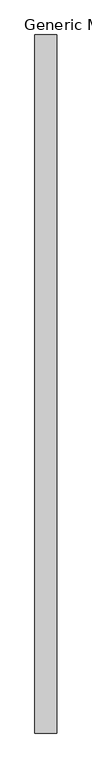
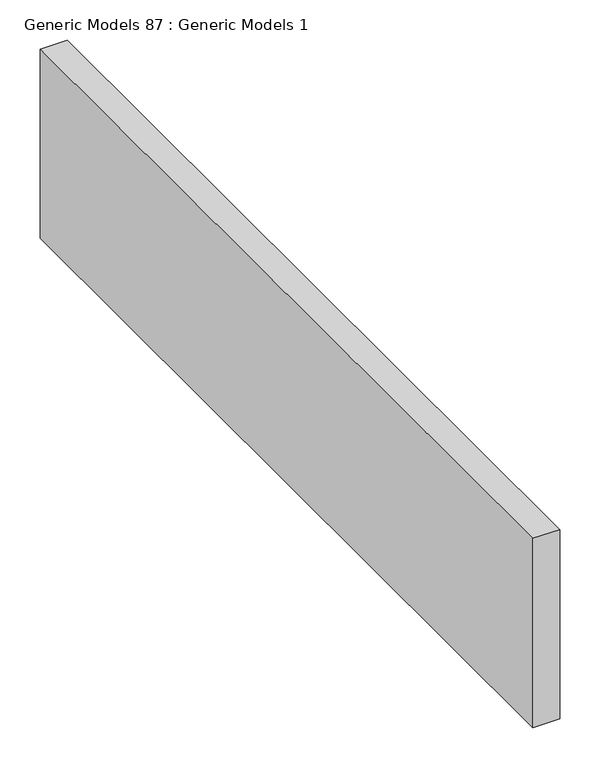
"""IFC4 building model written with IfcOpenShell, lengths in millimetres: proxy geometry, Generic Models 87 : Generic Models 1."""

import ifcopenshell
import ifcopenshell.guid

model = None  # the IFC model being written
_history = None  # IfcOwnerHistory: only IFC2X3 demands one
_inside = {}  # id of a spatial element -> (the spatial element, [elements in it])
_under = {}  # id of a project, library or spatial element -> (it, [spatial elements below it])
_declared = {}  # id of a project -> (the project, [libraries it declares])
_typed = {}  # id of a type object -> (the type object, [elements of that type])
_made_of = {}  # id of a material, layer set ... -> (it, [elements and type objects made of it])


def new_model(schema):
    """Start an empty IFC model of exactly this schema.

    Asked for "IFC4X3", IfcOpenShell would pick the latest addendum, in which some entities
    have other attributes; the version numbers below select the first issue.
    IFC2X3 requires an IfcOwnerHistory on every rooted entity: one is made here for all.
    """
    global model, _history
    if schema == "IFC4X3":
        model = ifcopenshell.file(schema_version=(4, 3, 0, 0))
    else:
        model = ifcopenshell.file(schema=schema)
    _inside.clear()
    _under.clear()
    _declared.clear()
    _typed.clear()
    _made_of.clear()
    _history = None
    if model.schema == "IFC2X3":
        org = make("IfcOrganization", Name="unknown")
        user = make(
            "IfcPersonAndOrganization",
            ThePerson=make("IfcPerson", FamilyName="unknown"),
            TheOrganization=org,
        )
        app = make(
            "IfcApplication",
            ApplicationDeveloper=org,
            Version="unknown",
            ApplicationFullName="unknown",
            ApplicationIdentifier="unknown",
        )
        _history = make(
            "IfcOwnerHistory",
            OwningUser=user,
            OwningApplication=app,
            ChangeAction="ADDED",
            CreationDate=0,
        )
    return model


def make(cls, **values):
    """One entity of the class cls with the attributes given. An attribute that is None is left unset."""
    return model.create_entity(
        cls, **{name: value for name, value in values.items() if value is not None}
    )


def rooted(cls, **values):
    """An entity with a GlobalId (a new one), such as an element, a storey or a relation."""
    return make(cls, GlobalId=ifcopenshell.guid.new(), OwnerHistory=_history, **values)


def si_unit(unit_type, name, prefix=None):
    """IfcSIUnit, for example si_unit("LENGTHUNIT", "METRE", prefix="MILLI")."""
    return make("IfcSIUnit", UnitType=unit_type, Prefix=prefix, Name=name)


def assignment(units):
    """IfcUnitAssignment: the units of a project."""
    return None if units is None else make("IfcUnitAssignment", Units=units)


def point(xyz):
    """IfcCartesianPoint."""
    return None if xyz is None else make("IfcCartesianPoint", Coordinates=xyz)


def direction(xyz):
    """IfcDirection."""
    return None if xyz is None else make("IfcDirection", DirectionRatios=xyz)


def frame(location, z_axis=None, x_axis=None):
    """IfcAxis2Placement3D, a coordinate frame: its origin and axes. An axis left out is left unset."""
    return make(
        "IfcAxis2Placement3D",
        Location=point(location),
        Axis=direction(z_axis),
        RefDirection=direction(x_axis),
    )


def origin():
    """The frame at (0, 0, 0) with its axes left unset."""
    return frame((0.0, 0.0, 0.0))


def place(relative_to, where):
    """IfcLocalPlacement: puts the frame where relative to a parent placement (None: the world)."""
    return make(
        "IfcLocalPlacement", PlacementRelTo=relative_to, RelativePlacement=where
    )


def context(
    kind, dimensions, precision=None, world=None, true_north=None, identifier=None
):
    """IfcGeometricRepresentationContext, for example the 3D "Model" context."""
    return make(
        "IfcGeometricRepresentationContext",
        ContextIdentifier=identifier,
        ContextType=kind,
        CoordinateSpaceDimension=dimensions,
        Precision=precision,
        WorldCoordinateSystem=world,
        TrueNorth=true_north,
    )


def project(units=None, contexts=None):
    """IfcProject with its units and contexts."""
    return rooted(
        "IfcProject",
        Name="project",
        RepresentationContexts=contexts,
        UnitsInContext=assignment(units),
    )


def spatial(cls, under=None, at=None, **own):
    """A site, building, storey or space (cls), placed at a placement, below another one or the project."""
    s = rooted(cls, ObjectPlacement=at, **own)
    if under is not None:
        _under.setdefault(under.id(), (under, []))[1].append(s)
    return s


def polyline(points):
    """IfcPolyline through the points."""
    return make("IfcPolyline", Points=[point(p) for p in points])


def outline(outer, holes=None, kind="AREA"):
    """IfcArbitraryClosedProfileDef: a profile drawn as a closed curve; with holes, ...WithVoids."""
    if holes is None:
        return make("IfcArbitraryClosedProfileDef", ProfileType=kind, OuterCurve=outer)
    return make(
        "IfcArbitraryProfileDefWithVoids",
        ProfileType=kind,
        OuterCurve=outer,
        InnerCurves=holes,
    )


def extrude(swept, where, along, depth):
    """IfcExtrudedAreaSolid: the profile swept, set in the frame where, extruded along a direction by depth."""
    return make(
        "IfcExtrudedAreaSolid",
        SweptArea=swept,
        Position=where,
        ExtrudedDirection=direction(along),
        Depth=depth,
    )


def shape(context_of_items, identifier, shape_type, items):
    """IfcShapeRepresentation: the items that make up one representation, for example the "Body"."""
    return make(
        "IfcShapeRepresentation",
        ContextOfItems=context_of_items,
        RepresentationIdentifier=identifier,
        RepresentationType=shape_type,
        Items=items,
    )


def source(mapping_origin, context_of_items, identifier, shape_type, items):
    """IfcRepresentationMap: a shape defined once, which mapped items show again and again."""
    return make(
        "IfcRepresentationMap",
        MappingOrigin=mapping_origin,
        MappedRepresentation=shape(context_of_items, identifier, shape_type, items),
    )


def transform(
    local_origin,
    x_axis=None,
    y_axis=None,
    z_axis=None,
    scale=None,
    scale2=None,
    scale3=None,
    uniform=True,
):
    """IfcCartesianTransformationOperator3D, or its non-uniform kind. x_axis, y_axis, z_axis: its Axis1, 2, 3."""
    if uniform:
        return make(
            "IfcCartesianTransformationOperator3D",
            Axis1=direction(x_axis),
            Axis2=direction(y_axis),
            LocalOrigin=point(local_origin),
            Scale=scale,
            Axis3=direction(z_axis),
        )
    return make(
        "IfcCartesianTransformationOperator3DnonUniform",
        Axis1=direction(x_axis),
        Axis2=direction(y_axis),
        LocalOrigin=point(local_origin),
        Scale=scale,
        Axis3=direction(z_axis),
        Scale2=scale2,
        Scale3=scale3,
    )


def mapped(mapping_source, mapping_target):
    """IfcMappedItem: shows the shape of a source again, moved by a transform."""
    return make(
        "IfcMappedItem", MappingSource=mapping_source, MappingTarget=mapping_target
    )


def made_of(thing, what):
    """Note that an element or type object is made of a material, layer set ...; save() writes the relation."""
    if what is not None:
        _made_of.setdefault(what.id(), (what, []))[1].append(thing)
    return thing


def element(
    cls,
    number,
    at=None,
    inside=None,
    cuts=None,
    type_object=None,
    material=None,
    context=None,
    identifier="Body",
    shape_type=None,
    held_by="IfcProductDefinitionShape",
    body=None,
    shapes=None,
    **own,
):
    """One element of the class cls, such as IfcWall. Its Tag is "e" and its number.

    at: its placement. inside: the storey or other place that contains it. cuts: it is an
    opening in that element (IfcRelVoidsElement). A single representation is given by context,
    identifier, shape_type and body (its items); several are given by shapes. held_by: the class
    of the entity that holds the representations. save() writes the other relations.
    """
    e = rooted(cls, Tag="e%d" % number, ObjectPlacement=at, **own)
    if body is not None:
        shapes = [shape(context, identifier, shape_type, body)]
    if shapes is not None:
        e.Representation = make(held_by, Representations=shapes)
    if inside is not None:
        _inside.setdefault(inside.id(), (inside, []))[1].append(e)
    if cuts is not None:
        rooted(
            "IfcRelVoidsElement", RelatingBuildingElement=cuts, RelatedOpeningElement=e
        )
    if type_object is not None:
        _typed.setdefault(type_object.id(), (type_object, []))[1].append(e)
    return made_of(e, material)


def aggregate(whole, parts):
    """IfcRelAggregates: a whole, such as a stair, and the parts it consists of."""
    return rooted("IfcRelAggregates", RelatingObject=whole, RelatedObjects=parts)


def save(model, path):
    """Write the relations noted so far, then the file.

    IfcRelAggregates (storeys below a building ...), IfcRelContainedInSpatialStructure (elements
    in a storey), IfcRelDefinesByType, IfcRelAssociatesMaterial and IfcRelDeclares: one each for
    every whole, place, type object, material and project.
    """
    for whole, parts in _under.values():
        aggregate(whole, parts)
    for where, things in _inside.values():
        rooted(
            "IfcRelContainedInSpatialStructure",
            RelatedElements=things,
            RelatingStructure=where,
        )
    for kind, things in _typed.values():
        rooted("IfcRelDefinesByType", RelatedObjects=things, RelatingType=kind)
    for what, things in _made_of.values():
        rooted("IfcRelAssociatesMaterial", RelatedObjects=things, RelatingMaterial=what)
    for by, libraries in _declared.values():
        rooted("IfcRelDeclares", RelatingContext=by, RelatedDefinitions=libraries)
    model.write(path)


def generic_models_87_generic_models_1_55a64953(model_context):
    return source(origin(), model_context, "Body", "SweptSolid", [
        extrude(outline(polyline([(51968.4, 0.0), (51930.3, 0.0), (51930.3, 1219.2), (51968.4, 1219.2), (51968.4, 0.0)])), frame((0.0, 0.0, 5222.478125), z_axis=(0.0, 0.0, 1.0), x_axis=(1.0, 0.0, 0.0)), (0.0, 0.0, 1.0), 285.75),
    ])


if __name__ == "__main__":
    model = new_model("IFC4")
    model_context = context("Model", 3, world=origin())
    ifc_project = project(units=[si_unit("LENGTHUNIT", "METRE", prefix="MILLI")], contexts=[model_context])
    site = spatial("IfcSite", under=ifc_project)
    building = spatial("IfcBuilding", under=site)
    placement = place(None, origin())
    generic_models_87_generic_models_1_shape = generic_models_87_generic_models_1_55a64953(model_context)
    element("IfcBuildingElementProxy", 1, Name="Generic Models 87 : Generic Models 1", ObjectType="Generic Models 87 : Generic Models 1", at=placement, inside=building, context=model_context, shape_type="MappedRepresentation", body=[
        mapped(generic_models_87_generic_models_1_shape, transform((0.0, 0.0, 0.0), x_axis=(1.0, 0.0, 0.0), y_axis=(0.0, 1.0, 0.0), z_axis=(0.0, 0.0, 1.0))),
    ])
    save(model, "model.ifc")

# Revit data of these elements
# Element 1 (IfcBuildingElementProxy, "Generic Models 87 : Generic Models 1")
#   Materials on its faces: "2X12 LEDGER WITH HILTI 3/8* DIAMETER HLC SLEEVE ANCHOR @ 8” OC."
# Materials
#   "2X12 LEDGER WITH HILTI 3/8* DIAMETER HLC SLEEVE ANCHOR @ 8” OC.": class "Wood", colour RGB 234 198 147, transparency 0, Description = "Pinus Echinata", Cost = 0
